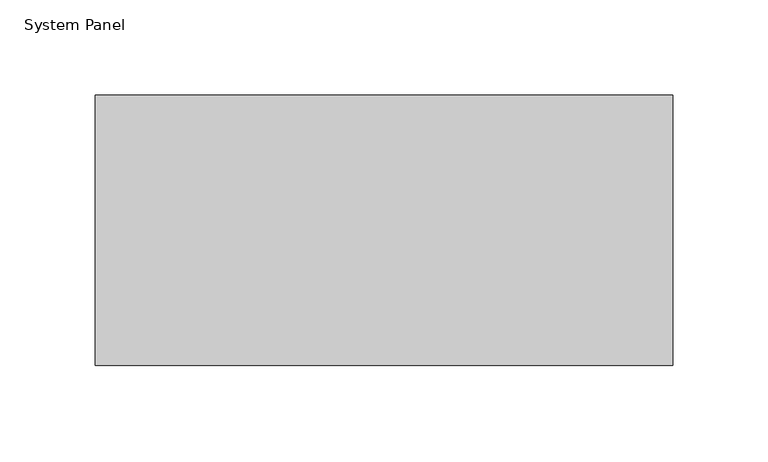
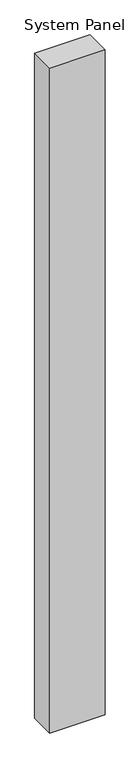
"""IFC4 building model written with IfcOpenShell, lengths in millimetres: plate geometry, System Panel : NLRS_21_CWP_hsb-vulling minerale wol 142 _gen_rsf."""

from ifc_helpers import new_model, si_unit, origin, origin_with_axes, place, context, project, spatial, polyline, outline, extrude, source, transform, mapped, element, save


def system_panel_d3f78fb4(model_context):
    return source(origin(), model_context, "Body", "SweptSolid", [
        extrude(outline(polyline([(151.4999998, -71.0), (-151.4999998, -71.0), (-151.4999998, 71.0), (151.4999998, 71.0), (151.4999998, -71.0)])), origin_with_axes(), (0.0, 0.0, 1.0), 3849.0),
    ])


if __name__ == "__main__":
    model = new_model("IFC4")
    model_context = context("Model", 3, world=origin())
    ifc_project = project(units=[si_unit("LENGTHUNIT", "METRE", prefix="MILLI")], contexts=[model_context])
    site = spatial("IfcSite", under=ifc_project)
    building = spatial("IfcBuilding", under=site)
    placement = place(None, origin())
    system_panel_shape = system_panel_d3f78fb4(model_context)
    element("IfcPlate", 1, ObjectType="System Panel : NLRS_21_CWP_hsb-vulling minerale wol 142 _gen_rsf", at=placement, inside=building, context=model_context, shape_type="MappedRepresentation", body=[
        mapped(system_panel_shape, transform((0.0, 0.0, 0.0), x_axis=(1.0, 0.0, 0.0), y_axis=(0.0, 1.0, 0.0), z_axis=(0.0, 0.0, 1.0))),
    ])
    save(model, "model.ifc")

# Revit data of these elements
# Type "System Panel : NLRS_21_CWP_hsb-vulling minerale wol 142 _gen_rsf"
#   Export Type to IFC As = "IfcWall"
#   Type IfcGUID = "07M7mRoiH1CR8m_RSKIwpC"
#   Assembly Code = "21.23"
# Element 1 (IfcPlate, "System Panel : NLRS_21_CWP_hsb-vulling minerale wol 142 _gen_rsf")
#   Materials on its faces: "NLRS_m1_isolatie minerale wol_gen_rsf"
# Materials
#   "NLRS_m1_isolatie minerale wol_gen_rsf": class "M - Anorganische materialen", colour RGB 200 200 140, transparency 0, Keynote = "m1", Manufacturer = "Revit Standards Foundation", URL = "www.revitstandards.org", Description = "isolatie minerale wol", Cost = 0
